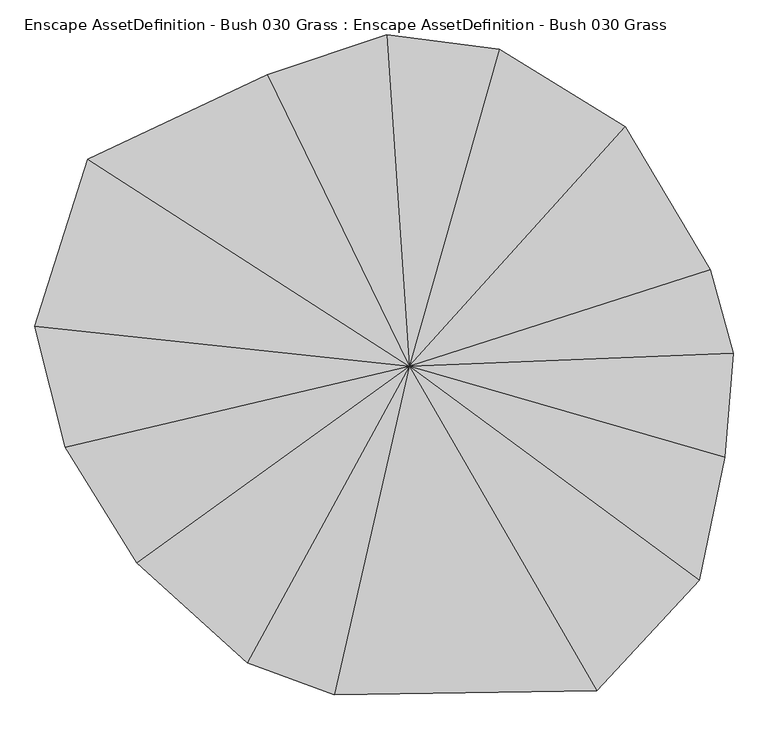
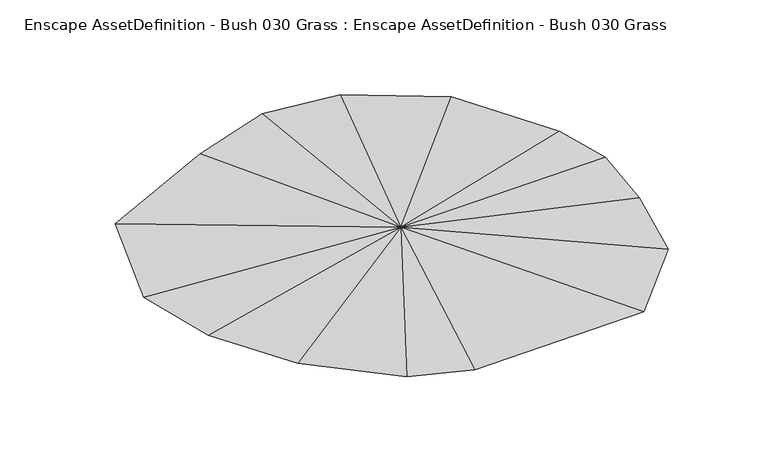
"""IFC4 building model written with IfcOpenShell, lengths in millimetres: geographic element geometry, Enscape AssetDefinition - Bush 030 Grass : Enscape AssetDefinition - Bush 030 Grass."""

import ifcopenshell
import ifcopenshell.guid

model = None  # the IFC model being written
_history = None  # IfcOwnerHistory: only IFC2X3 demands one
_inside = {}  # id of a spatial element -> (the spatial element, [elements in it])
_under = {}  # id of a project, library or spatial element -> (it, [spatial elements below it])
_declared = {}  # id of a project -> (the project, [libraries it declares])
_typed = {}  # id of a type object -> (the type object, [elements of that type])
_made_of = {}  # id of a material, layer set ... -> (it, [elements and type objects made of it])


def new_model(schema):
    """Start an empty IFC model of exactly this schema.

    Asked for "IFC4X3", IfcOpenShell would pick the latest addendum, in which some entities
    have other attributes; the version numbers below select the first issue.
    IFC2X3 requires an IfcOwnerHistory on every rooted entity: one is made here for all.
    """
    global model, _history
    if schema == "IFC4X3":
        model = ifcopenshell.file(schema_version=(4, 3, 0, 0))
    else:
        model = ifcopenshell.file(schema=schema)
    _inside.clear()
    _under.clear()
    _declared.clear()
    _typed.clear()
    _made_of.clear()
    _history = None
    if model.schema == "IFC2X3":
        org = make("IfcOrganization", Name="unknown")
        user = make(
            "IfcPersonAndOrganization",
            ThePerson=make("IfcPerson", FamilyName="unknown"),
            TheOrganization=org,
        )
        app = make(
            "IfcApplication",
            ApplicationDeveloper=org,
            Version="unknown",
            ApplicationFullName="unknown",
            ApplicationIdentifier="unknown",
        )
        _history = make(
            "IfcOwnerHistory",
            OwningUser=user,
            OwningApplication=app,
            ChangeAction="ADDED",
            CreationDate=0,
        )
    return model


def make(cls, **values):
    """One entity of the class cls with the attributes given. An attribute that is None is left unset."""
    return model.create_entity(
        cls, **{name: value for name, value in values.items() if value is not None}
    )


def rooted(cls, **values):
    """An entity with a GlobalId (a new one), such as an element, a storey or a relation."""
    return make(cls, GlobalId=ifcopenshell.guid.new(), OwnerHistory=_history, **values)


def si_unit(unit_type, name, prefix=None):
    """IfcSIUnit, for example si_unit("LENGTHUNIT", "METRE", prefix="MILLI")."""
    return make("IfcSIUnit", UnitType=unit_type, Prefix=prefix, Name=name)


def assignment(units):
    """IfcUnitAssignment: the units of a project."""
    return None if units is None else make("IfcUnitAssignment", Units=units)


def point(xyz):
    """IfcCartesianPoint."""
    return None if xyz is None else make("IfcCartesianPoint", Coordinates=xyz)


def direction(xyz):
    """IfcDirection."""
    return None if xyz is None else make("IfcDirection", DirectionRatios=xyz)


def frame(location, z_axis=None, x_axis=None):
    """IfcAxis2Placement3D, a coordinate frame: its origin and axes. An axis left out is left unset."""
    return make(
        "IfcAxis2Placement3D",
        Location=point(location),
        Axis=direction(z_axis),
        RefDirection=direction(x_axis),
    )


def origin():
    """The frame at (0, 0, 0) with its axes left unset."""
    return frame((0.0, 0.0, 0.0))


def place(relative_to, where):
    """IfcLocalPlacement: puts the frame where relative to a parent placement (None: the world)."""
    return make(
        "IfcLocalPlacement", PlacementRelTo=relative_to, RelativePlacement=where
    )


def context(
    kind, dimensions, precision=None, world=None, true_north=None, identifier=None
):
    """IfcGeometricRepresentationContext, for example the 3D "Model" context."""
    return make(
        "IfcGeometricRepresentationContext",
        ContextIdentifier=identifier,
        ContextType=kind,
        CoordinateSpaceDimension=dimensions,
        Precision=precision,
        WorldCoordinateSystem=world,
        TrueNorth=true_north,
    )


def project(units=None, contexts=None):
    """IfcProject with its units and contexts."""
    return rooted(
        "IfcProject",
        Name="project",
        RepresentationContexts=contexts,
        UnitsInContext=assignment(units),
    )


def spatial(cls, under=None, at=None, **own):
    """A site, building, storey or space (cls), placed at a placement, below another one or the project."""
    s = rooted(cls, ObjectPlacement=at, **own)
    if under is not None:
        _under.setdefault(under.id(), (under, []))[1].append(s)
    return s


def faces_of(points, faces, orient=None, outer=None):
    """IfcFace entities. A face is a list of loops; a loop is a list of indices into points, from 0.

    orient and outer hold one flag for each loop. By default every Orientation is true, the
    first loop of a face is its IfcFaceOuterBound and the others are IfcFaceBound.
    """
    made = []
    for i, loops in enumerate(faces):
        bounds = []
        for j, loop in enumerate(loops):
            is_outer = j == 0 if outer is None else outer[i][j]
            bounds.append(
                make(
                    "IfcFaceOuterBound" if is_outer else "IfcFaceBound",
                    Bound=make("IfcPolyLoop", Polygon=[points[k] for k in loop]),
                    Orientation=True if orient is None else orient[i][j],
                )
            )
        made.append(make("IfcFace", Bounds=bounds))
    return made


def faceted_brep(points, faces, orient=None, outer=None, voids=None):
    """IfcFacetedBrep: a solid bounded by flat faces; with voids (closed shells), ...WithVoids."""
    shared = [point(p) for p in points]
    hull = make("IfcClosedShell", CfsFaces=faces_of(shared, faces, orient, outer))
    if voids is None:
        return make("IfcFacetedBrep", Outer=hull)
    return make(
        "IfcFacetedBrepWithVoids",
        Outer=hull,
        Voids=[
            make(cls, CfsFaces=faces_of(shared, fs, o, b)) for cls, fs, o, b in voids
        ],
    )


def shape(context_of_items, identifier, shape_type, items):
    """IfcShapeRepresentation: the items that make up one representation, for example the "Body"."""
    return make(
        "IfcShapeRepresentation",
        ContextOfItems=context_of_items,
        RepresentationIdentifier=identifier,
        RepresentationType=shape_type,
        Items=items,
    )


def source(mapping_origin, context_of_items, identifier, shape_type, items):
    """IfcRepresentationMap: a shape defined once, which mapped items show again and again."""
    return make(
        "IfcRepresentationMap",
        MappingOrigin=mapping_origin,
        MappedRepresentation=shape(context_of_items, identifier, shape_type, items),
    )


def transform(
    local_origin,
    x_axis=None,
    y_axis=None,
    z_axis=None,
    scale=None,
    scale2=None,
    scale3=None,
    uniform=True,
):
    """IfcCartesianTransformationOperator3D, or its non-uniform kind. x_axis, y_axis, z_axis: its Axis1, 2, 3."""
    if uniform:
        return make(
            "IfcCartesianTransformationOperator3D",
            Axis1=direction(x_axis),
            Axis2=direction(y_axis),
            LocalOrigin=point(local_origin),
            Scale=scale,
            Axis3=direction(z_axis),
        )
    return make(
        "IfcCartesianTransformationOperator3DnonUniform",
        Axis1=direction(x_axis),
        Axis2=direction(y_axis),
        LocalOrigin=point(local_origin),
        Scale=scale,
        Axis3=direction(z_axis),
        Scale2=scale2,
        Scale3=scale3,
    )


def mapped(mapping_source, mapping_target):
    """IfcMappedItem: shows the shape of a source again, moved by a transform."""
    return make(
        "IfcMappedItem", MappingSource=mapping_source, MappingTarget=mapping_target
    )


def made_of(thing, what):
    """Note that an element or type object is made of a material, layer set ...; save() writes the relation."""
    if what is not None:
        _made_of.setdefault(what.id(), (what, []))[1].append(thing)
    return thing


def element(
    cls,
    number,
    at=None,
    inside=None,
    cuts=None,
    type_object=None,
    material=None,
    context=None,
    identifier="Body",
    shape_type=None,
    held_by="IfcProductDefinitionShape",
    body=None,
    shapes=None,
    **own,
):
    """One element of the class cls, such as IfcWall. Its Tag is "e" and its number.

    at: its placement. inside: the storey or other place that contains it. cuts: it is an
    opening in that element (IfcRelVoidsElement). A single representation is given by context,
    identifier, shape_type and body (its items); several are given by shapes. held_by: the class
    of the entity that holds the representations. save() writes the other relations.
    """
    e = rooted(cls, Tag="e%d" % number, ObjectPlacement=at, **own)
    if body is not None:
        shapes = [shape(context, identifier, shape_type, body)]
    if shapes is not None:
        e.Representation = make(held_by, Representations=shapes)
    if inside is not None:
        _inside.setdefault(inside.id(), (inside, []))[1].append(e)
    if cuts is not None:
        rooted(
            "IfcRelVoidsElement", RelatingBuildingElement=cuts, RelatedOpeningElement=e
        )
    if type_object is not None:
        _typed.setdefault(type_object.id(), (type_object, []))[1].append(e)
    return made_of(e, material)


def aggregate(whole, parts):
    """IfcRelAggregates: a whole, such as a stair, and the parts it consists of."""
    return rooted("IfcRelAggregates", RelatingObject=whole, RelatedObjects=parts)


def save(model, path):
    """Write the relations noted so far, then the file.

    IfcRelAggregates (storeys below a building ...), IfcRelContainedInSpatialStructure (elements
    in a storey), IfcRelDefinesByType, IfcRelAssociatesMaterial and IfcRelDeclares: one each for
    every whole, place, type object, material and project.
    """
    for whole, parts in _under.values():
        aggregate(whole, parts)
    for where, things in _inside.values():
        rooted(
            "IfcRelContainedInSpatialStructure",
            RelatedElements=things,
            RelatingStructure=where,
        )
    for kind, things in _typed.values():
        rooted("IfcRelDefinesByType", RelatedObjects=things, RelatingType=kind)
    for what, things in _made_of.values():
        rooted("IfcRelAssociatesMaterial", RelatedObjects=things, RelatingMaterial=what)
    for by, libraries in _declared.values():
        rooted("IfcRelDeclares", RelatingContext=by, RelatedDefinitions=libraries)
    model.write(path)


def enscape_assetdefinition_bush_030_grass_enscape_fc38328f(model_context):
    return source(origin(), model_context, "Body", "Brep", [
        faceted_brep([(46.6700345, 4.837607, 10.4857637), (-156.0632885, 421.6965139, 0.0005243), (-413.0132496, 301.0389209, 0.0), (14.2548708, 478.6814153, 0.0005243), (-488.4850383, 62.3530708, 0.0005243), (175.0823557, 458.5749507, 0.0), (355.5533588, 347.4667668, 0.0), (509.7507238, 23.7492062, 0.0005243), (-60.6722012, -464.8402035, 0.0), (-445.4378784, -110.6646508, 0.0), (-343.1681097, -275.8107185, 0.0), (-185.1303428, -419.0105796, 0.0005243), (315.0657415, -459.1831267, 0.0005243), (461.2535238, -301.1049926, 0.0), (498.0376065, -125.5266517, 0.0), (476.8353701, 142.9650038, 0.0)], [[[0, 1, 2]], [[0, 3, 1]], [[2, 1, 3]], [[0, 2, 4]], [[2, 3, 4]], [[0, 5, 3]], [[6, 3, 5]], [[7, 3, 6]], [[8, 3, 7]], [[4, 3, 8]], [[0, 4, 9]], [[4, 10, 9]], [[4, 8, 10]], [[0, 9, 10]], [[0, 10, 11]], [[10, 8, 11]], [[0, 11, 8]], [[0, 8, 12]], [[8, 13, 12]], [[8, 7, 13]], [[0, 12, 13]], [[0, 13, 14]], [[13, 7, 14]], [[0, 14, 7]], [[0, 7, 15]], [[0, 15, 6]], [[0, 6, 5]], [[7, 6, 15]]]),
    ])


if __name__ == "__main__":
    model = new_model("IFC4")
    model_context = context("Model", 3, world=origin())
    ifc_project = project(units=[si_unit("LENGTHUNIT", "METRE", prefix="MILLI")], contexts=[model_context])
    site = spatial("IfcSite", under=ifc_project)
    building = spatial("IfcBuilding", under=site)
    placement = place(None, origin())
    enscape_assetdefinition_bush_030_grass_enscape_shape = enscape_assetdefinition_bush_030_grass_enscape_fc38328f(model_context)
    element("IfcGeographicElement", 1, ObjectType="Enscape AssetDefinition - Bush 030 Grass : Enscape AssetDefinition - Bush 030 Grass", at=placement, inside=building, context=model_context, shape_type="MappedRepresentation", body=[
        mapped(enscape_assetdefinition_bush_030_grass_enscape_shape, transform((0.0, 0.0, 0.0), x_axis=(1.0, 0.0, 0.0), y_axis=(0.0, 1.0, 0.0), z_axis=(0.0, 0.0, 1.0))),
    ])
    save(model, "model.ifc")

# Revit data of these elements
# Type "Enscape AssetDefinition - Bush 030 Grass : Enscape AssetDefinition - Bush 030 Grass"
#   EnscapeAssetSource = "REMOTE"
#   EnscapeAssetId = "00026ee4-e1b1-4e5d-9a6f-71123b7d7688"
#   Height = 0.010486 m
#   EnscapeNativeAssetHeight = 0.010486 m
#   Default Elevation = 0
